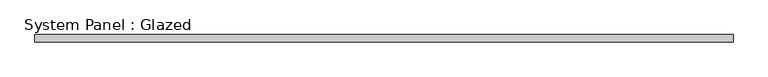
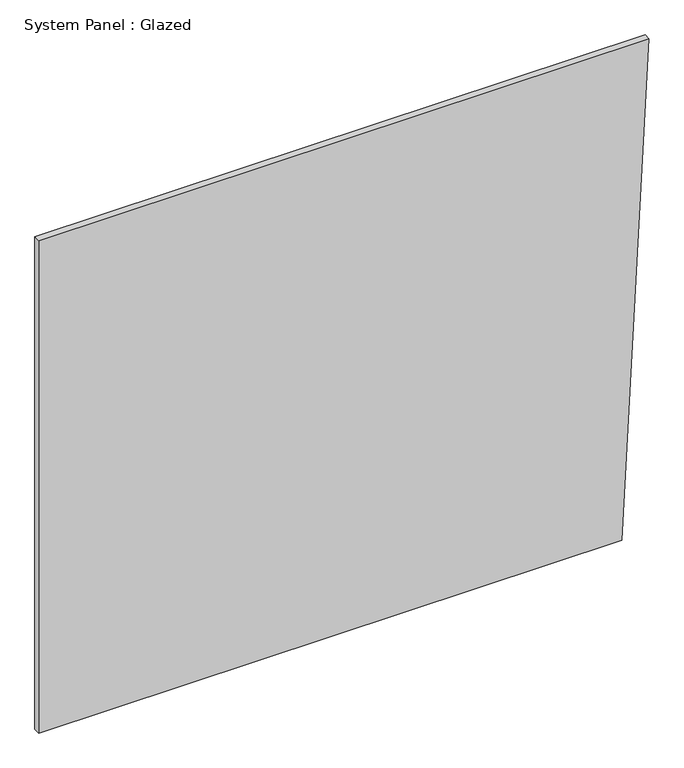
"""IFC4 building model written with IfcOpenShell, lengths in millimetres: plate geometry, System Panel : Glazed."""

import ifcopenshell
import ifcopenshell.guid

model = None  # the IFC model being written
_history = None  # IfcOwnerHistory: only IFC2X3 demands one
_inside = {}  # id of a spatial element -> (the spatial element, [elements in it])
_under = {}  # id of a project, library or spatial element -> (it, [spatial elements below it])
_declared = {}  # id of a project -> (the project, [libraries it declares])
_typed = {}  # id of a type object -> (the type object, [elements of that type])
_made_of = {}  # id of a material, layer set ... -> (it, [elements and type objects made of it])


def new_model(schema):
    """Start an empty IFC model of exactly this schema.

    Asked for "IFC4X3", IfcOpenShell would pick the latest addendum, in which some entities
    have other attributes; the version numbers below select the first issue.
    IFC2X3 requires an IfcOwnerHistory on every rooted entity: one is made here for all.
    """
    global model, _history
    if schema == "IFC4X3":
        model = ifcopenshell.file(schema_version=(4, 3, 0, 0))
    else:
        model = ifcopenshell.file(schema=schema)
    _inside.clear()
    _under.clear()
    _declared.clear()
    _typed.clear()
    _made_of.clear()
    _history = None
    if model.schema == "IFC2X3":
        org = make("IfcOrganization", Name="unknown")
        user = make(
            "IfcPersonAndOrganization",
            ThePerson=make("IfcPerson", FamilyName="unknown"),
            TheOrganization=org,
        )
        app = make(
            "IfcApplication",
            ApplicationDeveloper=org,
            Version="unknown",
            ApplicationFullName="unknown",
            ApplicationIdentifier="unknown",
        )
        _history = make(
            "IfcOwnerHistory",
            OwningUser=user,
            OwningApplication=app,
            ChangeAction="ADDED",
            CreationDate=0,
        )
    return model


def make(cls, **values):
    """One entity of the class cls with the attributes given. An attribute that is None is left unset."""
    return model.create_entity(
        cls, **{name: value for name, value in values.items() if value is not None}
    )


def rooted(cls, **values):
    """An entity with a GlobalId (a new one), such as an element, a storey or a relation."""
    return make(cls, GlobalId=ifcopenshell.guid.new(), OwnerHistory=_history, **values)


def si_unit(unit_type, name, prefix=None):
    """IfcSIUnit, for example si_unit("LENGTHUNIT", "METRE", prefix="MILLI")."""
    return make("IfcSIUnit", UnitType=unit_type, Prefix=prefix, Name=name)


def assignment(units):
    """IfcUnitAssignment: the units of a project."""
    return None if units is None else make("IfcUnitAssignment", Units=units)


def point(xyz):
    """IfcCartesianPoint."""
    return None if xyz is None else make("IfcCartesianPoint", Coordinates=xyz)


def direction(xyz):
    """IfcDirection."""
    return None if xyz is None else make("IfcDirection", DirectionRatios=xyz)


def frame(location, z_axis=None, x_axis=None):
    """IfcAxis2Placement3D, a coordinate frame: its origin and axes. An axis left out is left unset."""
    return make(
        "IfcAxis2Placement3D",
        Location=point(location),
        Axis=direction(z_axis),
        RefDirection=direction(x_axis),
    )


def origin():
    """The frame at (0, 0, 0) with its axes left unset."""
    return frame((0.0, 0.0, 0.0))


def place(relative_to, where):
    """IfcLocalPlacement: puts the frame where relative to a parent placement (None: the world)."""
    return make(
        "IfcLocalPlacement", PlacementRelTo=relative_to, RelativePlacement=where
    )


def context(
    kind, dimensions, precision=None, world=None, true_north=None, identifier=None
):
    """IfcGeometricRepresentationContext, for example the 3D "Model" context."""
    return make(
        "IfcGeometricRepresentationContext",
        ContextIdentifier=identifier,
        ContextType=kind,
        CoordinateSpaceDimension=dimensions,
        Precision=precision,
        WorldCoordinateSystem=world,
        TrueNorth=true_north,
    )


def project(units=None, contexts=None):
    """IfcProject with its units and contexts."""
    return rooted(
        "IfcProject",
        Name="project",
        RepresentationContexts=contexts,
        UnitsInContext=assignment(units),
    )


def spatial(cls, under=None, at=None, **own):
    """A site, building, storey or space (cls), placed at a placement, below another one or the project."""
    s = rooted(cls, ObjectPlacement=at, **own)
    if under is not None:
        _under.setdefault(under.id(), (under, []))[1].append(s)
    return s


def polyline(points):
    """IfcPolyline through the points."""
    return make("IfcPolyline", Points=[point(p) for p in points])


def outline(outer, holes=None, kind="AREA"):
    """IfcArbitraryClosedProfileDef: a profile drawn as a closed curve; with holes, ...WithVoids."""
    if holes is None:
        return make("IfcArbitraryClosedProfileDef", ProfileType=kind, OuterCurve=outer)
    return make(
        "IfcArbitraryProfileDefWithVoids",
        ProfileType=kind,
        OuterCurve=outer,
        InnerCurves=holes,
    )


def extrude(swept, where, along, depth):
    """IfcExtrudedAreaSolid: the profile swept, set in the frame where, extruded along a direction by depth."""
    return make(
        "IfcExtrudedAreaSolid",
        SweptArea=swept,
        Position=where,
        ExtrudedDirection=direction(along),
        Depth=depth,
    )


def shape(context_of_items, identifier, shape_type, items):
    """IfcShapeRepresentation: the items that make up one representation, for example the "Body"."""
    return make(
        "IfcShapeRepresentation",
        ContextOfItems=context_of_items,
        RepresentationIdentifier=identifier,
        RepresentationType=shape_type,
        Items=items,
    )


def source(mapping_origin, context_of_items, identifier, shape_type, items):
    """IfcRepresentationMap: a shape defined once, which mapped items show again and again."""
    return make(
        "IfcRepresentationMap",
        MappingOrigin=mapping_origin,
        MappedRepresentation=shape(context_of_items, identifier, shape_type, items),
    )


def transform(
    local_origin,
    x_axis=None,
    y_axis=None,
    z_axis=None,
    scale=None,
    scale2=None,
    scale3=None,
    uniform=True,
):
    """IfcCartesianTransformationOperator3D, or its non-uniform kind. x_axis, y_axis, z_axis: its Axis1, 2, 3."""
    if uniform:
        return make(
            "IfcCartesianTransformationOperator3D",
            Axis1=direction(x_axis),
            Axis2=direction(y_axis),
            LocalOrigin=point(local_origin),
            Scale=scale,
            Axis3=direction(z_axis),
        )
    return make(
        "IfcCartesianTransformationOperator3DnonUniform",
        Axis1=direction(x_axis),
        Axis2=direction(y_axis),
        LocalOrigin=point(local_origin),
        Scale=scale,
        Axis3=direction(z_axis),
        Scale2=scale2,
        Scale3=scale3,
    )


def mapped(mapping_source, mapping_target):
    """IfcMappedItem: shows the shape of a source again, moved by a transform."""
    return make(
        "IfcMappedItem", MappingSource=mapping_source, MappingTarget=mapping_target
    )


def made_of(thing, what):
    """Note that an element or type object is made of a material, layer set ...; save() writes the relation."""
    if what is not None:
        _made_of.setdefault(what.id(), (what, []))[1].append(thing)
    return thing


def element(
    cls,
    number,
    at=None,
    inside=None,
    cuts=None,
    type_object=None,
    material=None,
    context=None,
    identifier="Body",
    shape_type=None,
    held_by="IfcProductDefinitionShape",
    body=None,
    shapes=None,
    **own,
):
    """One element of the class cls, such as IfcWall. Its Tag is "e" and its number.

    at: its placement. inside: the storey or other place that contains it. cuts: it is an
    opening in that element (IfcRelVoidsElement). A single representation is given by context,
    identifier, shape_type and body (its items); several are given by shapes. held_by: the class
    of the entity that holds the representations. save() writes the other relations.
    """
    e = rooted(cls, Tag="e%d" % number, ObjectPlacement=at, **own)
    if body is not None:
        shapes = [shape(context, identifier, shape_type, body)]
    if shapes is not None:
        e.Representation = make(held_by, Representations=shapes)
    if inside is not None:
        _inside.setdefault(inside.id(), (inside, []))[1].append(e)
    if cuts is not None:
        rooted(
            "IfcRelVoidsElement", RelatingBuildingElement=cuts, RelatedOpeningElement=e
        )
    if type_object is not None:
        _typed.setdefault(type_object.id(), (type_object, []))[1].append(e)
    return made_of(e, material)


def aggregate(whole, parts):
    """IfcRelAggregates: a whole, such as a stair, and the parts it consists of."""
    return rooted("IfcRelAggregates", RelatingObject=whole, RelatedObjects=parts)


def save(model, path):
    """Write the relations noted so far, then the file.

    IfcRelAggregates (storeys below a building ...), IfcRelContainedInSpatialStructure (elements
    in a storey), IfcRelDefinesByType, IfcRelAssociatesMaterial and IfcRelDeclares: one each for
    every whole, place, type object, material and project.
    """
    for whole, parts in _under.values():
        aggregate(whole, parts)
    for where, things in _inside.values():
        rooted(
            "IfcRelContainedInSpatialStructure",
            RelatedElements=things,
            RelatingStructure=where,
        )
    for kind, things in _typed.values():
        rooted("IfcRelDefinesByType", RelatedObjects=things, RelatingType=kind)
    for what, things in _made_of.values():
        rooted("IfcRelAssociatesMaterial", RelatedObjects=things, RelatingMaterial=what)
    for by, libraries in _declared.values():
        rooted("IfcRelDeclares", RelatingContext=by, RelatedDefinitions=libraries)
    model.write(path)


def system_panel_glazed_7a24276e(model_context):
    return source(origin(), model_context, "Body", "SweptSolid", [
        extrude(outline(polyline([(0.0, -1222.0297486), (0.0, 1112.8894655), (2085.3785982, 1222.0297486), (2085.3785982, -1222.0297486), (0.0, -1222.0297486)])), frame((0.0, -44.45, 0.0), z_axis=(0.0, 1.0, 0.0), x_axis=(0.0, 0.0, 1.0)), (0.0, 0.0, 1.0), 25.4),
    ])


if __name__ == "__main__":
    model = new_model("IFC4")
    model_context = context("Model", 3, world=origin())
    ifc_project = project(units=[si_unit("LENGTHUNIT", "METRE", prefix="MILLI")], contexts=[model_context])
    site = spatial("IfcSite", under=ifc_project)
    building = spatial("IfcBuilding", under=site)
    placement = place(None, origin())
    system_panel_glazed_shape = system_panel_glazed_7a24276e(model_context)
    element("IfcPlate", 1, ObjectType="System Panel : Glazed", at=placement, inside=building, context=model_context, shape_type="MappedRepresentation", body=[
        mapped(system_panel_glazed_shape, transform((0.0, 0.0, 0.0), x_axis=(1.0, 0.0, 0.0), y_axis=(0.0, 1.0, 0.0), z_axis=(0.0, 0.0, 1.0))),
    ])
    save(model, "model.ifc")

# Revit data of these elements
# Type "System Panel : Glazed"
#   Construction Type Id = "GSP4R"
#   Analytic Construction = "1/8 in Pilkington single glazing"
#   Visual Light Transmittance = 0.9
#   Solar Heat Gain Coefficient = 0.86
#   Heat Transfer Coefficient (U) = 1.18115 BTU/(h·ft²·°F)
#   Define Thermal Properties by = 1
# Element 1 (IfcPlate, "System Panel : Glazed")
#   Materials on its faces: "Glass"
# Materials
#   "Glass": class "Glass", colour RGB 0 128 192, transparency 0.75, Description = "Soda Lime Glass", Cost = 0
